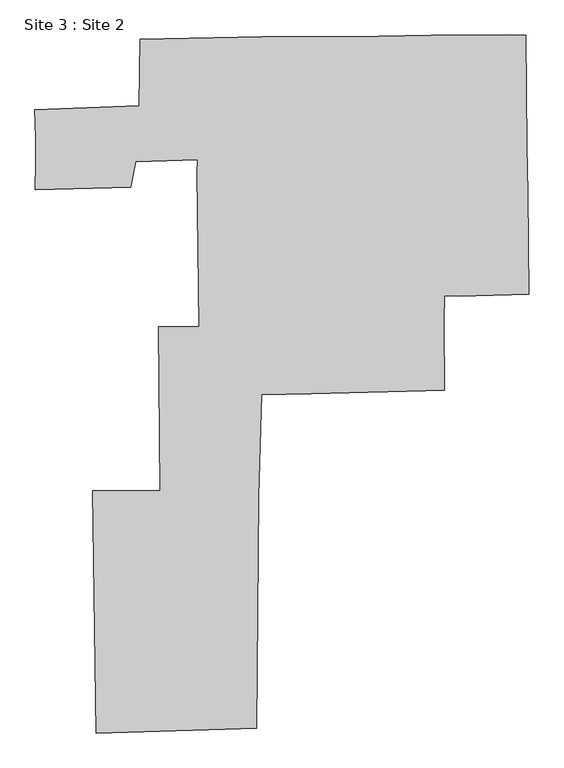
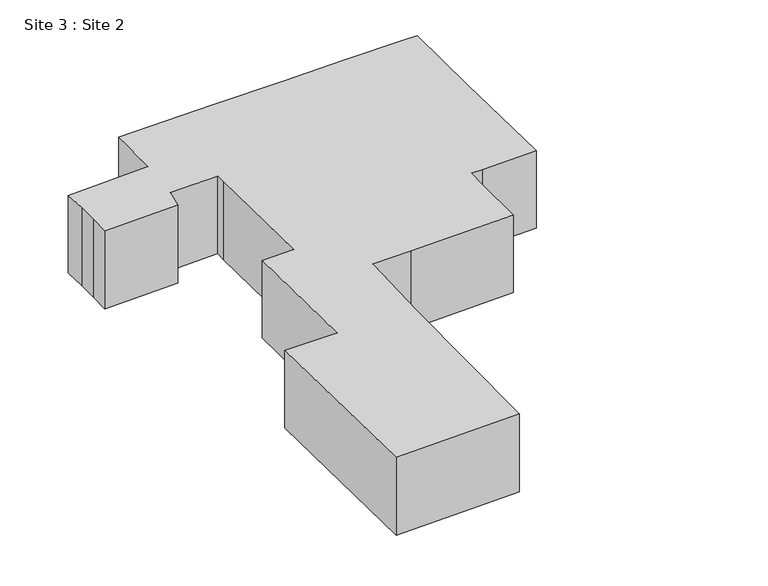
"""IFC4 building model written with IfcOpenShell, lengths in millimetres: geographic element geometry, Site 3 : Site 2."""

from ifc_helpers import new_model, si_unit, frame, origin, place, context, project, spatial, polyline, outline, extrude, source, transform, mapped, element, save


def site_3_site_2_de64f0c7(model_context):
    return source(origin(), model_context, "Body", "SweptSolid", [
        extrude(outline(polyline([(83491.7466699, 114170.3102481), (83588.9608665, 106853.0513744), (78506.5510943, 106723.4646024), (77490.6544407, 106738.1821473), (77464.1635221, 104909.613885), (77493.6401001, 99930.3306197), (67836.7646498, 99663.7983646), (64279.667343, 99613.7224622), (64072.1116969, 92300.8788642), (63930.8684085, 75537.446692), (52342.3235246, 75197.2905607), (52087.5161014, 92677.7195448), (56965.2756717, 92708.6626878), (56831.2256955, 104497.2268705), (59778.7875498, 104556.133263), (59634.4403957, 115633.6298325), (59647.685855, 116547.9139637), (55174.8115354, 116409.4967015), (54843.5507741, 114585.343715), (47931.0629269, 114380.6612878), (47959.0255632, 116310.8166757), (47985.5164818, 118139.384938), (47913.3594773, 120172.5992306), (55436.8587275, 120470.038232), (55506.0300726, 125244.6754669), (64348.7156358, 125421.3946446), (70851.9073121, 125428.7897526), (76543.8525367, 125549.5460344), (82234.3260436, 125568.7151906), (83351.8098229, 125552.5259279), (83438.7219955, 117524.1571745), (83491.7466699, 114170.3102481)])), frame((0.0, 0.0, 266395.2), z_axis=(0.0, 0.0, 1.0), x_axis=(1.0, 0.0, 0.0)), (0.0, 0.0, 1.0), 7620.0),
    ])


if __name__ == "__main__":
    model = new_model("IFC4")
    model_context = context("Model", 3, world=origin())
    ifc_project = project(units=[si_unit("LENGTHUNIT", "METRE", prefix="MILLI")], contexts=[model_context])
    site = spatial("IfcSite", under=ifc_project)
    building = spatial("IfcBuilding", under=site)
    placement = place(None, origin())
    site_3_site_2_shape = site_3_site_2_de64f0c7(model_context)
    element("IfcGeographicElement", 1, ObjectType="Site 3 : Site 2", at=placement, inside=building, context=model_context, shape_type="MappedRepresentation", body=[
        mapped(site_3_site_2_shape, transform((0.0, 0.0, 0.0), x_axis=(1.0, 0.0, 0.0), y_axis=(0.0, 1.0, 0.0), z_axis=(0.0, 0.0, 1.0))),
    ])
    save(model, "model.ifc")

# Revit data of these elements
# Element 1 (IfcGeographicElement, "Site 3 : Site 2")
#   Materials on its faces: "EXISTING BUILDING"
# Materials
#   "EXISTING BUILDING": class "Generic", colour RGB 120 120 120, transparency 0, Cost = 0
